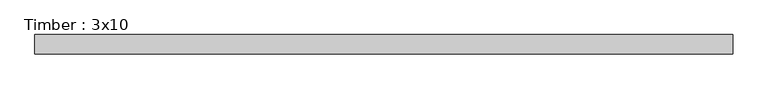
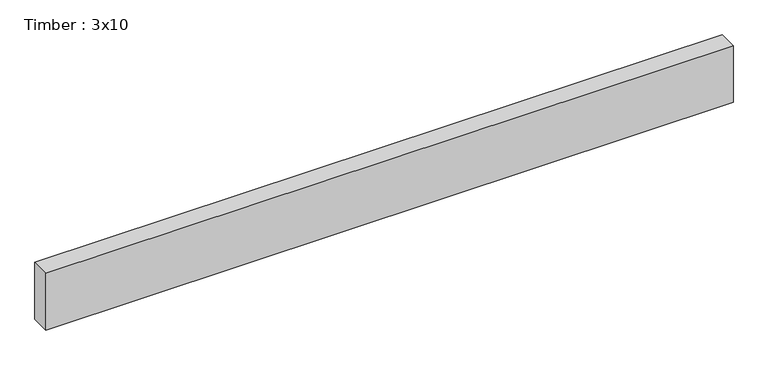
"""IFC4 building model written with IfcOpenShell, lengths in millimetres: beam geometry, Timber : 3x10."""

from ifc_helpers import new_model, si_unit, frame, origin, place, context, project, spatial, polyline, outline, extrude, source, transform, mapped, element, save


def timber_3x10_3e53af7a(model_context):
    return source(origin(), model_context, "Body", "SweptSolid", [
        extrude(outline(polyline([(1384.2999994, 38.1), (1384.2999994, -38.1), (-1384.3, -38.1), (-1384.3, 38.1), (1384.2999994, 38.1)])), frame((0.0, 0.0, -120.65), z_axis=(0.0, 0.0, 1.0), x_axis=(1.0, 0.0, 0.0)), (0.0, 0.0, 1.0), 241.3),
    ])


if __name__ == "__main__":
    model = new_model("IFC4")
    model_context = context("Model", 3, world=origin())
    ifc_project = project(units=[si_unit("LENGTHUNIT", "METRE", prefix="MILLI")], contexts=[model_context])
    site = spatial("IfcSite", under=ifc_project)
    building = spatial("IfcBuilding", under=site)
    placement = place(None, origin())
    timber_3x10_shape = timber_3x10_3e53af7a(model_context)
    element("IfcBeam", 1, ObjectType="Timber : 3x10", at=placement, inside=building, context=model_context, shape_type="MappedRepresentation", body=[
        mapped(timber_3x10_shape, transform((0.0, 0.0, 0.0), x_axis=(1.0, 0.0, 0.0), y_axis=(0.0, 1.0, 0.0), z_axis=(0.0, 0.0, 1.0))),
    ])
    save(model, "model.ifc")

# Revit data of these elements
# Type "Timber : 3x10"
#   Assembly Code = "B10"
#   A = 0.362847 SF
#   Length [instance default] = 5' - 0"
#   b = 0' - 3"
#   d = 0' - 9 1/2"
#   Structural Material [instance default] = Softwood, Lumber
# Element 1 (IfcBeam, "Timber : 3x10")
#   Materials on its faces: "Softwood, Lumber"
# Materials
#   "Softwood, Lumber": class "Wood", colour RGB 144 113 62, transparency 0, Description = "Pinus Echinata", Cost = 0
